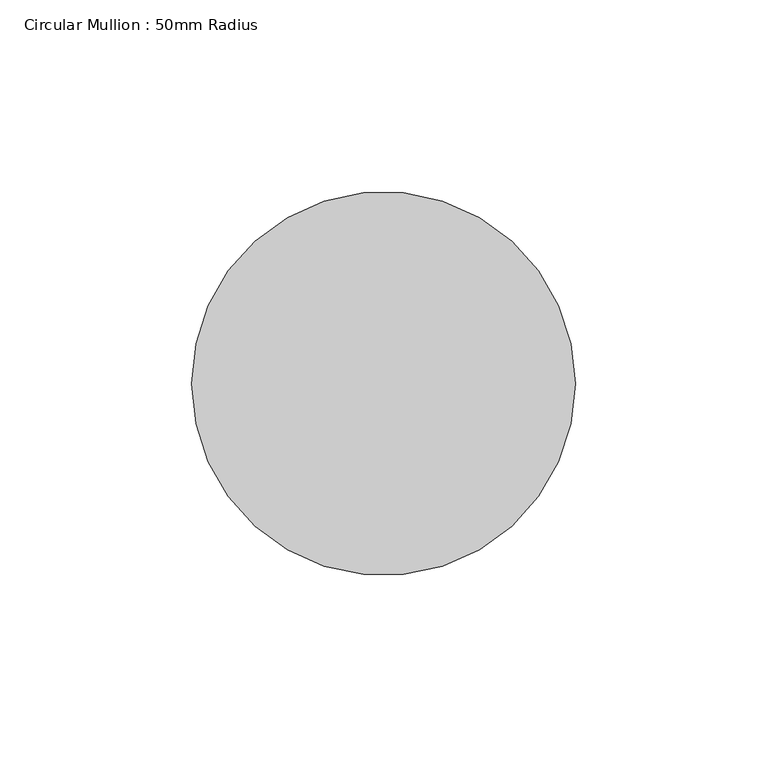
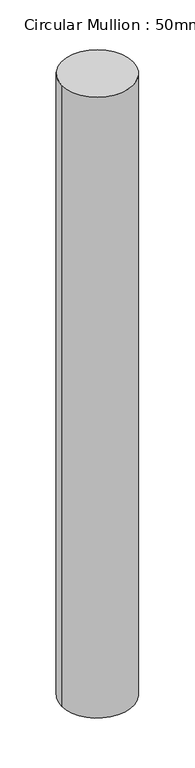
"""IFC4 building model written with IfcOpenShell, lengths in millimetres: member geometry, Circular Mullion : 50mm Radius."""

from ifc_helpers import new_model, si_unit, point, frame, origin, origin_2d, place, context, project, spatial, circle_curve, trimmed, segment, composite_curve, outline, extrude, source, transform, mapped, element, save


def circular_mullion_50mm_radius_d227ea2c(model_context):
    return source(origin(), model_context, "Body", "SweptSolid", [
        extrude(outline(composite_curve([segment(trimmed(circle_curve(origin_2d(), 50.0), [point((50.0, 0.0))], [point((-50.0, 0.0))], False, "CARTESIAN"), True, "CONTINUOUS"), segment(trimmed(circle_curve(origin_2d(), 50.0), [point((-50.0, 0.0))], [point((50.0, 0.0))], False, "CARTESIAN"), True, "CONTINUOUS")], self_intersect=False)), frame((0.0, 0.0, -918.8814436), z_axis=(0.0, 0.0, 1.0), x_axis=(1.0, 0.0, 0.0)), (0.0, 0.0, 1.0), 918.8814436),
    ])


if __name__ == "__main__":
    model = new_model("IFC4")
    model_context = context("Model", 3, world=origin())
    ifc_project = project(units=[si_unit("LENGTHUNIT", "METRE", prefix="MILLI")], contexts=[model_context])
    site = spatial("IfcSite", under=ifc_project)
    building = spatial("IfcBuilding", under=site)
    placement = place(None, origin())
    circular_mullion_50mm_radius_shape = circular_mullion_50mm_radius_d227ea2c(model_context)
    element("IfcMember", 1, ObjectType="Circular Mullion : 50mm Radius", at=placement, inside=building, context=model_context, shape_type="MappedRepresentation", body=[
        mapped(circular_mullion_50mm_radius_shape, transform((0.0, 0.0, 0.0), x_axis=(1.0, 0.0, 0.0), y_axis=(0.0, 1.0, 0.0), z_axis=(0.0, 0.0, 1.0))),
    ])
    save(model, "model.ifc")

# Revit data of these elements
# Type "Circular Mullion : 50mm Radius"
#   built-in parameter 1007350 = 0.164042 (stored number, unit not read)
# Element 1 (IfcMember, "Circular Mullion : 50mm Radius")
#   Materials on its faces: "Aluminium"
# Materials
#   "Aluminium": class "Metal", colour RGB 247 247 247, transparency 0, Description = "Aluminium 6061", Cost = 0
